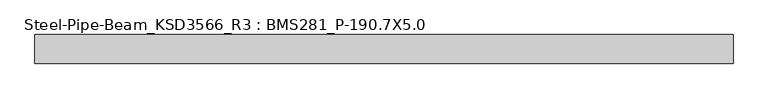
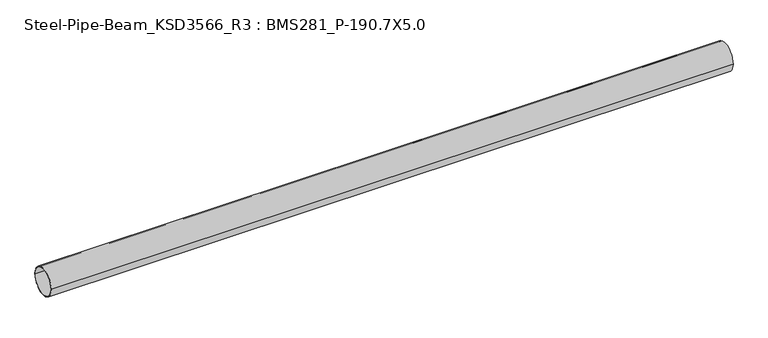
"""IFC4 building model written with IfcOpenShell, lengths in millimetres: member geometry, Steel-Pipe-Beam_KSD3566_R3 : BMS281_P-190.7X5.0."""

from ifc_helpers import new_model, si_unit, point, frame, origin, origin_2d, place, context, project, spatial, circle_curve, trimmed, segment, composite_curve, outline, extrude, source, transform, mapped, element, save


def steel_pipe_beam_ksd3566_r3_bms281_p_190_7x5_0_cf2b3cb5(model_context):
    return source(origin(), model_context, "Body", "SweptSolid", [
        extrude(outline(composite_curve([segment(trimmed(circle_curve(origin_2d(), 95.35), [point((-95.35, 0.0))], [point((95.35, 0.0))], False, "CARTESIAN"), True, "CONTINUOUS"), segment(trimmed(circle_curve(origin_2d(), 95.35), [point((95.35, 0.0))], [point((-95.35, 0.0))], False, "CARTESIAN"), True, "CONTINUOUS")], self_intersect=False), holes=[composite_curve([segment(trimmed(circle_curve(origin_2d(), 90.35), [point((90.35, 0.0))], [point((-90.35, 0.0))], True, "CARTESIAN"), True, "CONTINUOUS"), segment(trimmed(circle_curve(origin_2d(), 90.35), [point((-90.35, 0.0))], [point((90.35, 0.0))], True, "CARTESIAN"), True, "CONTINUOUS")], self_intersect=False)]), frame((-2342.207694, 0.0, 0.0), z_axis=(1.0, 0.0, 0.0), x_axis=(0.0, 1.0, 0.0)), (0.0, 0.0, 1.0), 4645.3125886),
    ])


if __name__ == "__main__":
    model = new_model("IFC4")
    model_context = context("Model", 3, world=origin())
    ifc_project = project(units=[si_unit("LENGTHUNIT", "METRE", prefix="MILLI")], contexts=[model_context])
    site = spatial("IfcSite", under=ifc_project)
    building = spatial("IfcBuilding", under=site)
    placement = place(None, origin())
    steel_pipe_beam_ksd3566_r3_bms281_p_190_7x5_0_shape = steel_pipe_beam_ksd3566_r3_bms281_p_190_7x5_0_cf2b3cb5(model_context)
    element("IfcMember", 1, ObjectType="Steel-Pipe-Beam_KSD3566_R3 : BMS281_P-190.7X5.0", at=placement, inside=building, context=model_context, shape_type="MappedRepresentation", body=[
        mapped(steel_pipe_beam_ksd3566_r3_bms281_p_190_7x5_0_shape, transform((0.0, 0.0, 0.0), x_axis=(1.0, 0.0, 0.0), y_axis=(0.0, 1.0, 0.0), z_axis=(0.0, 0.0, 1.0))),
    ])
    save(model, "model.ifc")

# Revit data of these elements
# Type "Steel-Pipe-Beam_KSD3566_R3 : BMS281_P-190.7X5.0"
#   Keynote = "P-190.7X5.0"
#   SteelWeight = "Light"
#   t = 0.0050 m
#   Surface Area = 0.599102 m²/m
#   Section Area = 29.1697 cm²
#   Mass per Unit Length = 22.8982 kg/m
#   Length [instance default] = 1.5000 m
#   D = 0.1907 m
#   hec_material4 [instance default] = none
#   hec_material3 [instance default] = none
#   hec_material2 [instance default] = none
#   hec_material1 [instance default] = none
#   Structural Material [instance default] = Steel, 45-345
#   Assembly Code = ""
# Element 1 (IfcMember, "Steel-Pipe-Beam_KSD3566_R3 : BMS281_P-190.7X5.0")
#   Structural Material = none
# Materials
#   "Steel, 45-345": class "Metal", colour RGB 189 187 185, transparency 0, Description = "Steel 345 MPa", Cost = 0
